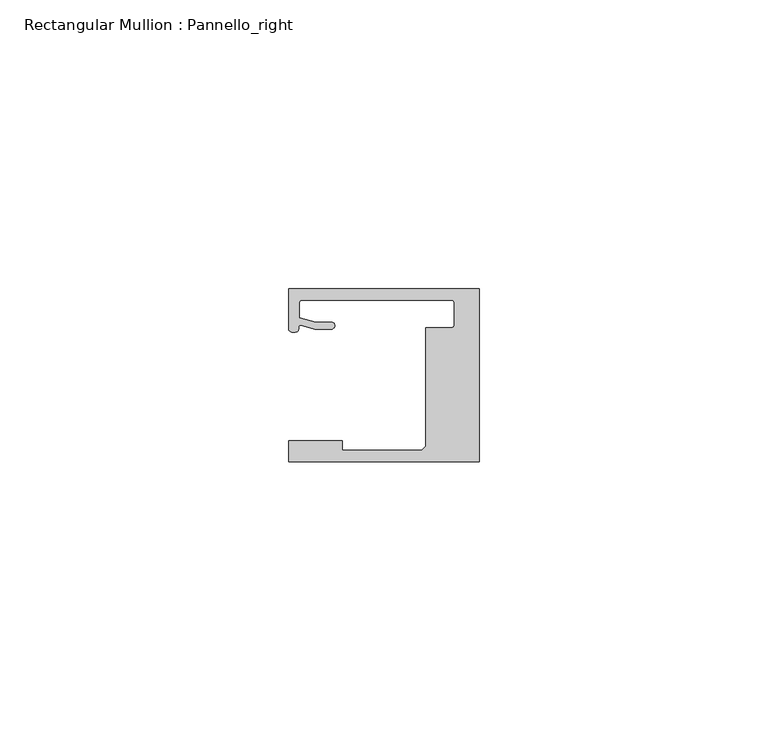
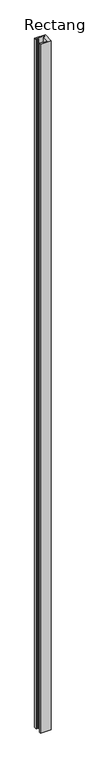
"""IFC4 building model written with IfcOpenShell, lengths in millimetres: member geometry, Rectangular Mullion : Pannello_right."""

from ifc_helpers import new_model, si_unit, frame, origin, place, context, project, spatial, polyline, circle_curve, source, transform, mapped, element, save
from ifc_brep_helpers import plane_surface, cylinder_surface, revolved_surface, extruded_surface, spline_curve, advanced_brep


def rectangular_mullion_pannello_right_610047ba(model_context):
    return source(origin(), model_context, "Body", "AdvancedBrep", [
        advanced_brep(
        [(-33.0, -15.0, 0.0), (0.0, -15.0, 0.0), (0.0, 15.0, 0.0), (-33.0000135, 15.0, 0.0), (-33.0000135, 8.0000472, 0.0), (-30.9223017, 8.6490241, 0.0), (-28.4999305, 7.9999523, 0.0), (-25.59998, 7.9999523, 0.0), (-25.59998, 9.1999523, 0.0), (-28.3419477, 9.1999523, 0.0), (-31.19998, 9.9657591, 0.0), (-31.19998, 12.50001, 0.0), (-30.69998, 13.00001, 0.0), (-4.7999726, 13.00001, 0.0), (-4.2999726, 12.50001, 0.0), (-4.2999726, 8.7500595, 0.0), (-4.7999726, 8.2500595, 0.0), (-9.2999726, 8.2500595, 0.0), (-9.2999726, -12.2999849, 0.0), (-10.0000103, -13.0000004, 0.0), (-23.700041, -13.0000004, 0.0), (-23.700041, -11.3000004, 0.0), (-33.0, -11.3000004, 0.0), (-33.0, -15.0, -2240.0), (-33.0, -11.3000004, -2240.0), (-23.700041, -11.3000004, -2240.0), (-23.700041, -13.0000004, -2240.0), (-10.0000103, -13.0000004, -2240.0), (-9.2999726, -12.2999849, -2240.0), (-9.2999726, 8.2500595, -2240.0), (-4.7999726, 8.2500595, -2240.0), (-4.2999726, 8.7500595, -2240.0), (-4.2999726, 12.50001, -2240.0), (-4.7999726, 13.00001, -2240.0), (-30.69998, 13.00001, -2240.0), (-31.19998, 12.50001, -2240.0), (-31.19998, 9.9657591, -2240.0), (-28.3419477, 9.1999523, -2240.0), (-25.59998, 9.1999523, -2240.0), (-25.59998, 7.9999523, -2240.0), (-28.4999305, 7.9999523, -2240.0), (-30.9223017, 8.6490241, -2240.0), (-33.0000135, 8.0000472, -2240.0), (-33.0000135, 15.0, -2240.0), (0.0, 15.0, -2240.0), (0.0, -15.0, -2240.0)],
        [
            (0, 1),
            (1, 2),
            (2, 3),
            (3, 4),
            (4, 5, spline_curve(3, [(-33.0000135, 8.0000472, 0.0), (-33.0000135, 7.457047519, 0.0), (-32.262327879, 7.456527435, 0.0), (-31.357433266, 7.563996614, 0.0), (-31.305645054, 7.690065204, 0.0), (-31.298563602, 8.366228555, 0.0), (-31.312054066, 8.717747958, 0.0), (-30.9223017, 8.6490241, 0.0)], [4, 2, 2, 4], [0.0, 0.0027053965905959043, 0.0058611956533709, 0.007702013405570312])),
            (5, 6),
            (6, 7),
            (7, 8, circle_curve(frame((-25.59998, 8.5999523, 0.0), z_axis=(0.0, 0.0, 1.0), x_axis=(0.0, 1.0, 0.0)), 0.6)),
            (8, 9),
            (9, 10),
            (10, 11),
            (11, 12, circle_curve(frame((-30.69998, 12.50001, 0.0), z_axis=(0.0, 0.0, -1.0), x_axis=(0.0, 1.0, 0.0)), 0.5)),
            (12, 13),
            (13, 14, circle_curve(frame((-4.7999726, 12.50001, 0.0), z_axis=(0.0, 0.0, -1.0), x_axis=(1.0, 0.0, 0.0)), 0.5)),
            (14, 15),
            (15, 16, circle_curve(frame((-4.7999726, 8.7500595, 0.0), z_axis=(0.0, 0.0, -1.0), x_axis=(0.0, -1.0, 0.0)), 0.5)),
            (16, 17),
            (17, 18),
            (18, 19),
            (19, 20),
            (20, 21),
            (21, 22),
            (22, 0),
            (23, 24),
            (24, 25),
            (25, 26),
            (26, 27),
            (27, 28),
            (28, 29),
            (29, 30),
            (30, 31, circle_curve(frame((-4.7999726, 8.7500595, -2240.0), z_axis=(0.0, 0.0, 1.0), x_axis=(0.0, -1.0, 0.0)), 0.5)),
            (31, 32),
            (32, 33, circle_curve(frame((-4.7999726, 12.50001, -2240.0), z_axis=(0.0, 0.0, 1.0), x_axis=(1.0, 0.0, 0.0)), 0.5)),
            (33, 34),
            (34, 35, circle_curve(frame((-30.69998, 12.50001, -2240.0), z_axis=(0.0, 0.0, 1.0), x_axis=(0.0, 1.0, 0.0)), 0.5)),
            (35, 36),
            (36, 37),
            (37, 38),
            (38, 39, circle_curve(frame((-25.59998, 8.5999523, -2240.0), z_axis=(0.0, 0.0, -1.0), x_axis=(0.0, 1.0, 0.0)), 0.6)),
            (39, 40),
            (40, 41),
            (41, 42, spline_curve(3, [(-30.9223017, 8.6490241, -2240.0), (-31.312054066, 8.717747958, -2240.0), (-31.298563602, 8.366228555, -2240.0), (-31.305645054, 7.690065204, -2240.0), (-31.357433266, 7.563996614, -2240.0), (-32.262327879, 7.456527435, -2240.0), (-33.0000135, 7.457047519, -2240.0), (-33.0000135, 8.0000472, -2240.0)], [4, 2, 2, 4], [0.0, 0.001840817752199412, 0.004996616814974408, 0.007702013405570312])),
            (42, 43),
            (43, 44),
            (44, 45),
            (45, 23),
            (0, 23),
            (45, 1),
            (44, 2),
            (43, 3),
            (42, 4),
            (41, 5),
            (40, 6),
            (39, 7),
            (38, 8),
            (37, 9),
            (36, 10),
            (35, 11),
            (34, 12),
            (33, 13),
            (32, 14),
            (31, 15),
            (30, 16),
            (29, 17),
            (28, 18),
            (27, 19),
            (26, 20),
            (25, 21),
            (24, 22),
        ],
        [
            plane_surface(frame((0.0, -36.2491502, 0.0), z_axis=(0.0, 0.0, 1.0), x_axis=(-1.0, 0.0, 0.0))),
            plane_surface(frame((0.0, -36.2491502, -2240.0), z_axis=(0.0, 0.0, -1.0), x_axis=(-1.0, 0.0, 0.0))),
            plane_surface(frame((-33.0, -15.0, 0.0), z_axis=(0.0, -1.0, 0.0), x_axis=(0.0, 0.0, -1.0))),
            plane_surface(frame((0.0, -15.0, 0.0), z_axis=(1.0, 0.0, 0.0), x_axis=(0.0, 0.0, -1.0))),
            plane_surface(frame((0.0, 15.0, 0.0), z_axis=(0.0, 1.0, 0.0), x_axis=(0.0, 0.0, -1.0))),
            plane_surface(frame((-33.0000135, 15.0, 0.0), z_axis=(-1.0, 0.0, 0.0), x_axis=(0.0, 0.0, -1.0))),
            extruded_surface(spline_curve(3, [(-33.0000135, 8.0000472, -2240.0), (-33.0000135, 7.457047519, -2240.0), (-32.262327879, 7.456527435, -2240.0), (-31.357433266, 7.563996614, -2240.0), (-31.305645054, 7.690065204, -2240.0), (-31.298563602, 8.366228555, -2240.0), (-31.312054066, 8.717747958, -2240.0), (-30.9223017, 8.6490241, -2240.0)], [4, 2, 2, 4], [0.0, 0.0027053965905959043, 0.0058611956533709, 0.007702013405570312]), (0.0, 0.0, 2240.0), 2240.0),
            plane_surface(frame((-30.9223017, 8.6490241, 0.0), z_axis=(-0.2588188320019168, -0.965925883389178, 0.0), x_axis=(0.0, 0.0, -1.0))),
            plane_surface(frame((-28.4999305, 7.9999523, 0.0), z_axis=(0.0, -1.0, 0.0), x_axis=(0.0, 0.0, -1.0))),
            cylinder_surface(frame((-25.59998, 8.5999523, 0.0), z_axis=(0.0, 0.0, 1.0), x_axis=(0.0, 1.0, 0.0)), 0.6),
            plane_surface(frame((-25.59998, 9.1999523, 0.0), z_axis=(0.0, 1.0, 0.0), x_axis=(0.0, 0.0, -1.0))),
            plane_surface(frame((-28.3419477, 9.1999523, 0.0), z_axis=(0.2588188320428738, 0.9659258833782035, 0.0), x_axis=(0.0, 0.0, -1.0))),
            plane_surface(frame((-31.19998, 9.9657591, 0.0), z_axis=(1.0, 0.0, 0.0), x_axis=(0.0, 0.0, -1.0))),
            revolved_surface(polyline([(-30.69998, 13.00001, -2240.0), (-30.69998, 13.00001, 0.0)]), (-30.69998, 12.50001, 0.0), (0.0, 0.0, -1.0)),
            plane_surface(frame((-30.69998, 13.00001, 0.0), z_axis=(0.0, -1.0, 0.0), x_axis=(0.0, 0.0, -1.0))),
            revolved_surface(polyline([(-4.2999726, 12.50001, -2240.0), (-4.2999726, 12.50001, 0.0)]), (-4.7999726, 12.50001, 0.0), (0.0, 0.0, -1.0)),
            plane_surface(frame((-4.2999726, 12.50001, 0.0), z_axis=(-1.0, 0.0, 0.0), x_axis=(0.0, 0.0, -1.0))),
            revolved_surface(polyline([(-4.7999726, 8.2500595, -2240.0), (-4.7999726, 8.2500595, 0.0)]), (-4.7999726, 8.7500595, 0.0), (0.0, 0.0, -1.0)),
            plane_surface(frame((-4.7999726, 8.2500595, 0.0), z_axis=(0.0, 1.0, 0.0), x_axis=(0.0, 0.0, -1.0))),
            plane_surface(frame((-9.2999726, 8.2500595, 0.0), z_axis=(-1.0, 0.0, 0.0), x_axis=(0.0, 0.0, -1.0))),
            plane_surface(frame((-9.2999726, -12.2999849, 0.0), z_axis=(-0.7070955486278075, 0.7071180135668587, 0.0), x_axis=(0.0, 0.0, -1.0))),
            plane_surface(frame((-10.0000103, -13.0000004, 0.0), z_axis=(0.0, 1.0, 0.0), x_axis=(0.0, 0.0, -1.0))),
            plane_surface(frame((-23.700041, -13.0000004, 0.0), z_axis=(1.0, 0.0, 0.0), x_axis=(0.0, 0.0, -1.0))),
            plane_surface(frame((-23.700041, -11.3000004, 0.0), z_axis=(0.0, 1.0, 0.0), x_axis=(0.0, 0.0, -1.0))),
            plane_surface(frame((-33.0, -11.3000004, 0.0), z_axis=(-1.0, 0.0, 0.0), x_axis=(0.0, 0.0, -1.0))),
        ],
        [
            (0, [[1, 2, 3, 4, 5, 6, 7, 8, 9, 10, 11, 12, 13, 14, 15, 16, 17, 18, 19, 20, 21, 22, 23]]),
            (1, [[24, 25, 26, 27, 28, 29, 30, 31, 32, 33, 34, 35, 36, 37, 38, 39, 40, 41, 42, 43, 44, 45, 46]]),
            (2, [[-1, 47, -46, 48]]),
            (3, [[-2, -48, -45, 49]]),
            (4, [[-3, -49, -44, 50]]),
            (5, [[-4, -50, -43, 51]]),
            (6, [[-5, -51, -42, 52]]),
            (7, [[-6, -52, -41, 53]]),
            (8, [[-7, -53, -40, 54]]),
            (9, [[-8, -54, -39, 55]]),
            (10, [[-9, -55, -38, 56]]),
            (11, [[-10, -56, -37, 57]]),
            (12, [[-11, -57, -36, 58]]),
            (13, [[-12, -58, -35, 59]]),
            (14, [[-13, -59, -34, 60]]),
            (15, [[-14, -60, -33, 61]]),
            (16, [[-15, -61, -32, 62]]),
            (17, [[-16, -62, -31, 63]]),
            (18, [[-17, -63, -30, 64]]),
            (19, [[-18, -64, -29, 65]]),
            (20, [[-19, -65, -28, 66]]),
            (21, [[-20, -66, -27, 67]]),
            (22, [[-21, -67, -26, 68]]),
            (23, [[-22, -68, -25, 69]]),
            (24, [[-23, -69, -24, -47]]),
        ],
    ),
    ])


if __name__ == "__main__":
    model = new_model("IFC4")
    model_context = context("Model", 3, world=origin())
    ifc_project = project(units=[si_unit("LENGTHUNIT", "METRE", prefix="MILLI")], contexts=[model_context])
    site = spatial("IfcSite", under=ifc_project)
    building = spatial("IfcBuilding", under=site)
    placement = place(None, origin())
    rectangular_mullion_pannello_right_shape = rectangular_mullion_pannello_right_610047ba(model_context)
    element("IfcMember", 1, ObjectType="Rectangular Mullion : Pannello_right", at=placement, inside=building, context=model_context, shape_type="MappedRepresentation", body=[
        mapped(rectangular_mullion_pannello_right_shape, transform((0.0, 0.0, 0.0), x_axis=(1.0, 0.0, 0.0), y_axis=(0.0, 1.0, 0.0), z_axis=(0.0, 0.0, 1.0))),
    ])
    save(model, "model.ifc")

# Revit data of these elements
# Type "Rectangular Mullion : Pannello_right"
#   built-in parameter 1007322 = 0.0984252 (stored number, unit not read)
#   built-in parameter 1007321 = 0.0305117 (stored number, unit not read)
#   built-in parameter 1007320 = 0 (stored number, unit not read)
